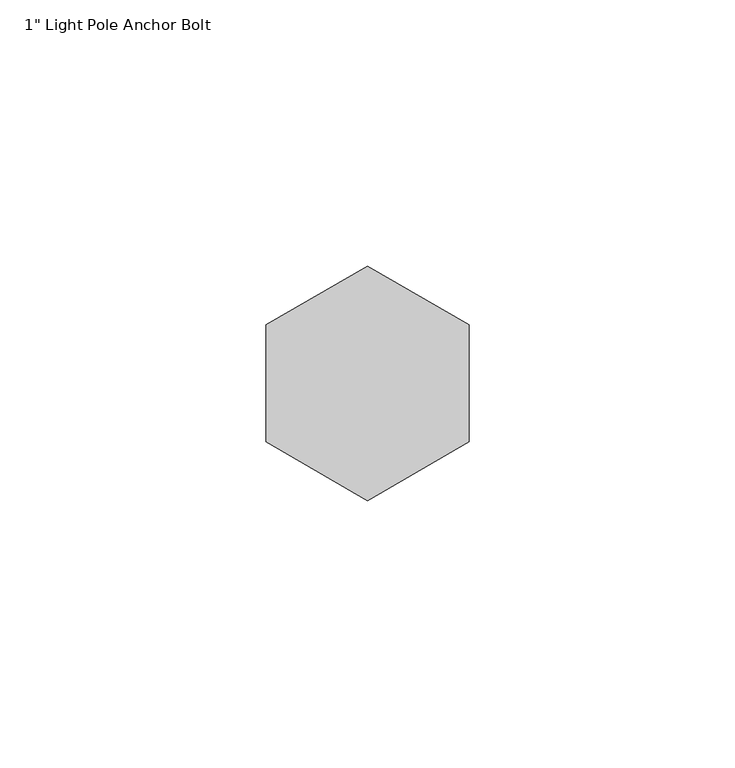
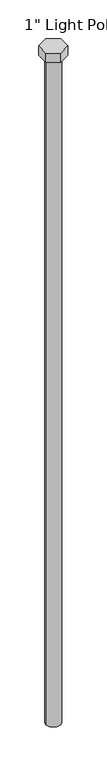
"""IFC4 building model written with IfcOpenShell, lengths in millimetres: proxy geometry."""

from ifc_helpers import new_model, si_unit, point, frame, origin, origin_with_axes, origin_2d, place, context, project, spatial, polyline, circle_curve, trimmed, segment, composite_curve, outline, extrude, source, transform, mapped, element, save


def proxy_d7e644cf(model_context):
    return source(origin(), model_context, "Body", "SweptSolid", [
        extrude(outline(polyline([(-19.05, -10.9985226), (-19.05, 10.9985226), (0.0, 21.9970453), (19.05, 10.9985226), (19.05, -10.9985226), (0.0, -21.9970453), (-19.05, -10.9985226)])), origin_with_axes(), (0.0, 0.0, 1.0), 17.065625),
        extrude(outline(composite_curve([segment(trimmed(circle_curve(origin_2d(), 12.7), [point((-12.7, 0.0))], [point((12.7, 0.0))], False, "CARTESIAN"), True, "CONTINUOUS"), segment(trimmed(circle_curve(origin_2d(), 12.7), [point((12.7, 0.0))], [point((-12.7, 0.0))], False, "CARTESIAN"), True, "CONTINUOUS")], self_intersect=False)), frame((0.0, 0.0, -1219.2), z_axis=(0.0, 0.0, 1.0), x_axis=(1.0, 0.0, 0.0)), (0.0, 0.0, 1.0), 1219.2),
    ])


if __name__ == "__main__":
    model = new_model("IFC4")
    model_context = context("Model", 3, world=origin())
    ifc_project = project(units=[si_unit("LENGTHUNIT", "METRE", prefix="MILLI")], contexts=[model_context])
    site = spatial("IfcSite", under=ifc_project)
    building = spatial("IfcBuilding", under=site)
    placement = place(None, origin())
    proxy_shape = proxy_d7e644cf(model_context)
    element("IfcBuildingElementProxy", 1, Name="050523 - W_P_C - Fastenings - Lag Bolt or Thru Bolt : 1\" Light Pole Anchor Bolt", ObjectType="050523 - W_P_C - Fastenings - Lag Bolt or Thru Bolt : 1\" Light Pole Anchor Bolt", at=placement, inside=building, context=model_context, shape_type="MappedRepresentation", body=[
        mapped(proxy_shape, transform((0.0, 0.0, 0.0), x_axis=(1.0, 0.0, 0.0), y_axis=(0.0, 1.0, 0.0), z_axis=(0.0, 0.0, 1.0))),
    ])
    save(model, "model.ifc")

# Revit data of these elements
# Type "050523 - W_P_C - Fastenings - Lag Bolt or Thru Bolt : 1\" Light Pole Anchor Bolt"
#   Thickness_of_Substrate [instance default] = 0' - 1"
#   Side = 0' - 0 111/128"
#   Radius = 0' - 0 1/2"
#   Length = 4' - 0"
#   Head Size = 0' - 1 1/2"
#   Head Radius = 0' - 0 3/4"
#   Head Height = 0' - 0 43/64"
#   Diameter = 0' - 1"
#   Default Elevation = 4' - 0"
#   Nut_Visibility [instance default] = yes
#   Bolt Material (Size) = (4) GALV. ANCHOR BOLTS - SUPPLIED W/ LIGHT POLE
# Element 1 (IfcBuildingElementProxy, "050523 - W_P_C - Fastenings - Lag Bolt or Thru Bolt : 1\" Light Pole Anchor Bolt")
#   Thickness_of_Substrate = 3' - 0"
#   Nut_Visibility = no
#   Materials on its faces: "(4) GALV. ANCHOR BOLTS - SUPPLIED W/ LIGHT POLE"
# Materials
#   "(4) GALV. ANCHOR BOLTS - SUPPLIED W/ LIGHT POLE": class "Generic", colour RGB 120 120 120, transparency 0, Cost = 0
